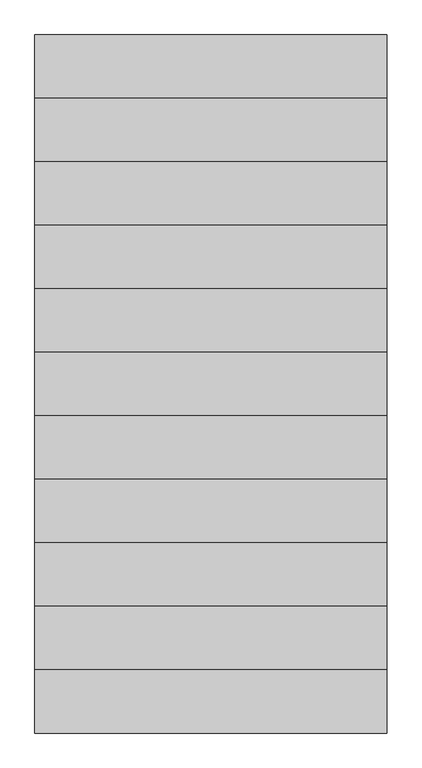
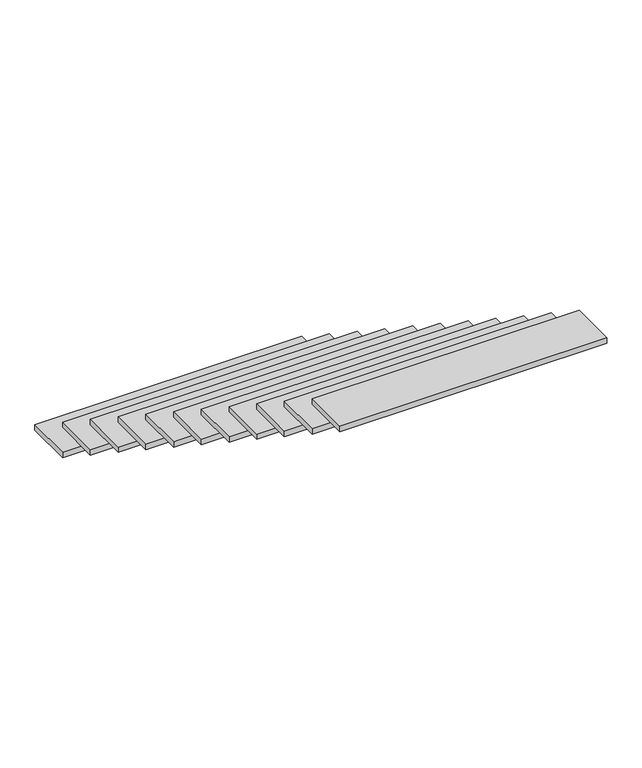
"""IFC4 building model written with IfcOpenShell, lengths in millimetres: stair flight geometry."""

from ifc_helpers import new_model, si_unit, frame, origin, place, context, project, spatial, polyline, outline, extrude, source, transform, mapped, element, save


def stair_flight_27635be5(model_context):
    return source(origin(), model_context, "Body", "SweptSolid", [
        extrude(outline(polyline([(16085.3403387, 4647.6066446), (14585.3403387, 4647.6066446), (14585.3403387, 4917.6066446), (16085.3403387, 4917.6066446), (16085.3403387, 4647.6066446)])), frame((0.0, 0.0, 2117.4505495), z_axis=(0.0, 0.0, 1.0), x_axis=(1.0, 0.0, 0.0)), (0.0, 0.0, 1.0), 32.0),
        extrude(outline(polyline([(16085.3403387, 4377.6066446), (14585.3403387, 4377.6066446), (14585.3403387, 4647.6066446), (16085.3403387, 4647.6066446), (16085.3403387, 4377.6066446)])), frame((0.0, 0.0, 2296.5714286), z_axis=(0.0, 0.0, 1.0), x_axis=(1.0, 0.0, 0.0)), (0.0, 0.0, 1.0), 32.0),
        extrude(outline(polyline([(16085.3403387, 4107.6066446), (14585.3403387, 4107.6066446), (14585.3403387, 4377.6066446), (16085.3403387, 4377.6066446), (16085.3403387, 4107.6066446)])), frame((0.0, 0.0, 2475.6923077), z_axis=(0.0, 0.0, 1.0), x_axis=(1.0, 0.0, 0.0)), (0.0, 0.0, 1.0), 32.0),
        extrude(outline(polyline([(16085.3403387, 3837.6066446), (14585.3403387, 3837.6066446), (14585.3403387, 4107.6066446), (16085.3403387, 4107.6066446), (16085.3403387, 3837.6066446)])), frame((0.0, 0.0, 2654.8131868), z_axis=(0.0, 0.0, 1.0), x_axis=(1.0, 0.0, 0.0)), (0.0, 0.0, 1.0), 32.0),
        extrude(outline(polyline([(16085.3403387, 3567.6066446), (14585.3403387, 3567.6066446), (14585.3403387, 3837.6066446), (16085.3403387, 3837.6066446), (16085.3403387, 3567.6066446)])), frame((0.0, 0.0, 2833.9340659), z_axis=(0.0, 0.0, 1.0), x_axis=(1.0, 0.0, 0.0)), (0.0, 0.0, 1.0), 32.0),
        extrude(outline(polyline([(16085.3403387, 3297.6066446), (14585.3403387, 3297.6066446), (14585.3403387, 3567.6066446), (16085.3403387, 3567.6066446), (16085.3403387, 3297.6066446)])), frame((0.0, 0.0, 3013.0549451), z_axis=(0.0, 0.0, 1.0), x_axis=(1.0, 0.0, 0.0)), (0.0, 0.0, 1.0), 32.0),
        extrude(outline(polyline([(16085.3403387, 3027.6066446), (14585.3403387, 3027.6066446), (14585.3403387, 3297.6066446), (16085.3403387, 3297.6066446), (16085.3403387, 3027.6066446)])), frame((0.0, 0.0, 3192.1758242), z_axis=(0.0, 0.0, 1.0), x_axis=(1.0, 0.0, 0.0)), (0.0, 0.0, 1.0), 32.0),
        extrude(outline(polyline([(16085.3403387, 2757.6066446), (14585.3403387, 2757.6066446), (14585.3403387, 3027.6066446), (16085.3403387, 3027.6066446), (16085.3403387, 2757.6066446)])), frame((0.0, 0.0, 3371.2967033), z_axis=(0.0, 0.0, 1.0), x_axis=(1.0, 0.0, 0.0)), (0.0, 0.0, 1.0), 32.0),
        extrude(outline(polyline([(16085.3403387, 2487.6066446), (14585.3403387, 2487.6066446), (14585.3403387, 2757.6066446), (16085.3403387, 2757.6066446), (16085.3403387, 2487.6066446)])), frame((0.0, 0.0, 3550.4175824), z_axis=(0.0, 0.0, 1.0), x_axis=(1.0, 0.0, 0.0)), (0.0, 0.0, 1.0), 32.0),
        extrude(outline(polyline([(16085.3403387, 2217.6066446), (14585.3403387, 2217.6066446), (14585.3403387, 2487.6066446), (16085.3403387, 2487.6066446), (16085.3403387, 2217.6066446)])), frame((0.0, 0.0, 3729.5384615), z_axis=(0.0, 0.0, 1.0), x_axis=(1.0, 0.0, 0.0)), (0.0, 0.0, 1.0), 32.0),
        extrude(outline(polyline([(16085.3403387, 1947.6066446), (14585.3403387, 1947.6066446), (14585.3403387, 2217.6066446), (16085.3403387, 2217.6066446), (16085.3403387, 1947.6066446)])), frame((0.0, 0.0, 3908.6593407), z_axis=(0.0, 0.0, 1.0), x_axis=(1.0, 0.0, 0.0)), (0.0, 0.0, 1.0), 32.0),
    ])


if __name__ == "__main__":
    model = new_model("IFC4")
    model_context = context("Model", 3, world=origin())
    ifc_project = project(units=[si_unit("LENGTHUNIT", "METRE", prefix="MILLI")], contexts=[model_context])
    site = spatial("IfcSite", under=ifc_project)
    building = spatial("IfcBuilding", under=site)
    placement = place(None, origin())
    stair_flight_shape = stair_flight_27635be5(model_context)
    element("IfcStairFlight", 1, at=placement, inside=building, context=model_context, shape_type="MappedRepresentation", body=[
        mapped(stair_flight_shape, transform((0.0, 0.0, 0.0), x_axis=(1.0, 0.0, 0.0), y_axis=(0.0, 1.0, 0.0), z_axis=(0.0, 0.0, 1.0))),
    ])
    save(model, "model.ifc")

# Revit data of these elements
# Element 1 (IfcStairFlight)
#   Materials on its faces: "철강"
# Materials
#   "철강": class "Generic", colour RGB 143 142 141, transparency 0, Description = "철골+가공조립+세우기", Cost = 0
